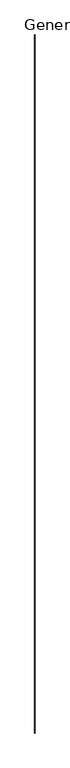
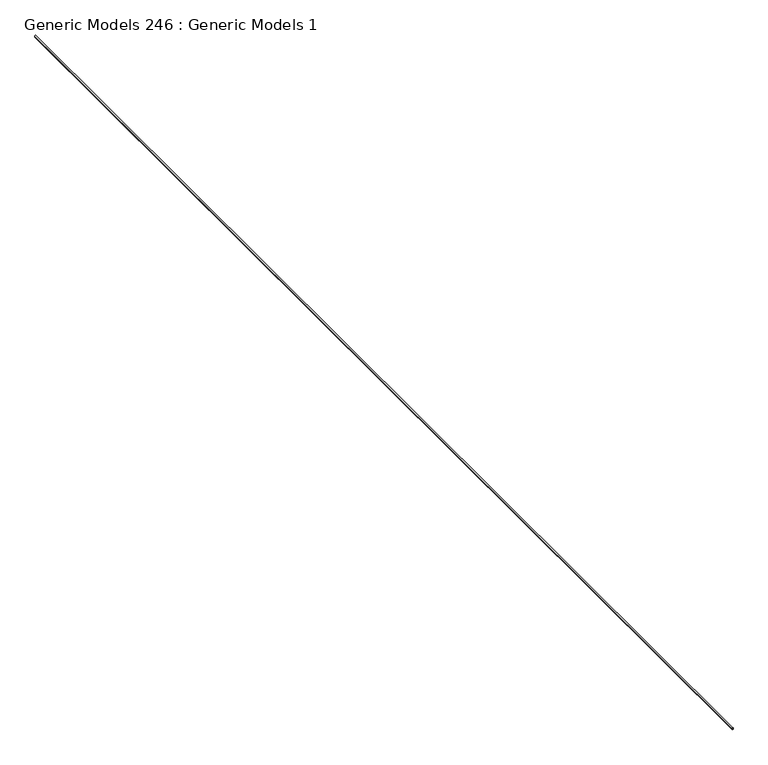
"""IFC4 building model written with IfcOpenShell, lengths in millimetres: proxy geometry, Generic Models 246 : Generic Models 1."""

from ifc_helpers import new_model, si_unit, point, frame, origin, place, context, project, spatial, polyline, circle_curve, ellipse_curve, trimmed, source, transform, mapped, element, save
from ifc_brep_helpers import plane_surface, cylinder_surface, revolved_surface, extruded_surface, advanced_brep


def generic_models_246_generic_models_1_4ee7912a(model_context):
    return source(origin(), model_context, "Body", "AdvancedBrep", [
        advanced_brep(
        [(2120.1002046, 306.6963299, 129317.7733897), (2120.1002046, 306.6963299, 129320.9483897), (2118.829546, 306.6963299, 129321.900149), (2115.0208631, 306.6963299, 129321.900149), (2113.7502046, 306.6963299, 129320.9483897), (2113.7502046, 306.6963299, 129317.7733897), (2120.1002046, 8193.3963299, 129317.7733897), (2113.7502046, 8193.3963299, 129317.7733897), (2113.7502046, 8193.3963299, 129320.9483897), (2115.0208631, 8193.3963299, 129321.900149), (2118.829546, 8193.3963299, 129321.900149), (2120.1002046, 8193.3963299, 129320.9483897)],
        [
            (0, 1),
            (1, 2, circle_curve(frame((2116.9252046, 306.6963299, 129318.0336492), z_axis=(0.0, -1.0, 0.0), x_axis=(1.0, 0.0, 0.0)), 4.3100275)),
            (2, 3, ellipse_curve(frame((2116.9252046, 306.6963299, 129325.7108897), z_axis=(0.0, -1.0, 0.0), x_axis=(0.0, 0.0, -1.0)), 4.7625, 3.175)),
            (3, 4, circle_curve(frame((2116.9252046, 306.6963299, 129318.0336492), z_axis=(0.0, -1.0, 0.0), x_axis=(1.0, 0.0, 0.0)), 4.3100275)),
            (4, 5),
            (5, 0, circle_curve(frame((2116.9252046, 306.6963299, 129314.8586492), z_axis=(0.0, 1.0, 0.0), x_axis=(1.0, 0.0, 0.0)), 4.3100275)),
            (6, 7, circle_curve(frame((2116.9252046, 8193.3963299, 129314.8586492), z_axis=(0.0, -1.0, 0.0), x_axis=(1.0, 0.0, 0.0)), 4.3100275)),
            (7, 8),
            (8, 9, circle_curve(frame((2116.9252046, 8193.3963299, 129318.0336492), z_axis=(0.0, 1.0, 0.0), x_axis=(1.0, 0.0, 0.0)), 4.3100275)),
            (9, 10, ellipse_curve(frame((2116.9252046, 8193.3963299, 129325.7108897), z_axis=(0.0, 1.0, 0.0), x_axis=(0.0, 0.0, -1.0)), 4.7625, 3.175)),
            (10, 11, circle_curve(frame((2116.9252046, 8193.3963299, 129318.0336492), z_axis=(0.0, 1.0, 0.0), x_axis=(1.0, 0.0, 0.0)), 4.3100275)),
            (11, 6),
            (2, 10),
            (9, 3),
            (0, 6),
            (11, 1),
            (8, 4),
            (7, 5),
        ],
        [
            plane_surface(frame((2113.7502046, 306.6963299, 129317.7733897), z_axis=(0.0, -1.0, 0.0), x_axis=(0.0, 0.0, 1.0))),
            plane_surface(frame((2113.7502046, 8193.3963299, 129317.7733897), z_axis=(0.0, 1.0, 0.0), x_axis=(0.0, 0.0, 1.0))),
            extruded_surface(trimmed(ellipse_curve(frame((2116.9252046, 8193.3963299, 129325.7108897), z_axis=(0.0, -1.0, 0.0), x_axis=(0.0, 0.0, -1.0)), 4.7625, 3.175), [point((2118.829546, 8193.3963299, 129321.900149))], [point((2115.0208631, 8193.3963299, 129321.900149))], True, "CARTESIAN"), (0.0, -7886.700000000001, 0.0), 7886.700000000001),
            plane_surface(frame((2120.1002046, 306.6963299, 129317.7733897), z_axis=(1.0, 0.0, 0.0), x_axis=(0.0, 1.0, 0.0))),
            cylinder_surface(frame((2116.9252046, 306.6963299, 129318.0336492), z_axis=(0.0, -1.0, 0.0), x_axis=(1.0, 0.0, 0.0)), 4.3100275),
            plane_surface(frame((2113.7502046, 306.6963299, 129320.9483897), z_axis=(-1.0, 0.0, 0.0), x_axis=(0.0, 1.0, 0.0))),
            revolved_surface(polyline([(2121.2352321000003, 8193.3963299, 129314.8586492), (2121.2352321000003, 306.6963299, 129314.8586492)]), (2116.9252046, 306.6963299, 129314.8586492), (0.0, 1.0, 0.0)),
        ],
        [
            (0, [[1, 2, 3, 4, 5, 6]]),
            (1, [[7, 8, 9, 10, 11, 12]]),
            (2, [[-3, 13, -10, 14]]),
            (3, [[-1, 15, -12, 16]]),
            (4, [[-4, -14, -9, 17]]),
            (5, [[-5, -17, -8, 18]]),
            (6, [[-6, -18, -7, -15]]),
            (4, [[-2, -16, -11, -13]]),
        ],
    ),
    ])


if __name__ == "__main__":
    model = new_model("IFC4")
    model_context = context("Model", 3, world=origin())
    ifc_project = project(units=[si_unit("LENGTHUNIT", "METRE", prefix="MILLI")], contexts=[model_context])
    site = spatial("IfcSite", under=ifc_project)
    building = spatial("IfcBuilding", under=site)
    placement = place(None, origin())
    generic_models_246_generic_models_1_shape = generic_models_246_generic_models_1_4ee7912a(model_context)
    element("IfcBuildingElementProxy", 1, Name="Generic Models 246 : Generic Models 1", ObjectType="Generic Models 246 : Generic Models 1", at=placement, inside=building, context=model_context, shape_type="MappedRepresentation", body=[
        mapped(generic_models_246_generic_models_1_shape, transform((0.0, 0.0, 0.0), x_axis=(1.0, 0.0, 0.0), y_axis=(0.0, 1.0, 0.0), z_axis=(0.0, 0.0, 1.0))),
    ])
    save(model, "model.ifc")

# Revit data of these elements
# Element 1 (IfcBuildingElementProxy, "Generic Models 246 : Generic Models 1")
#   Materials on its faces: "_SEALANT AND BACKROD, IF NECESSARY"
# Materials
#   "_SEALANT AND BACKROD, IF NECESSARY": class "Generic", colour RGB 190 220 196, transparency 0, Cost = 0
